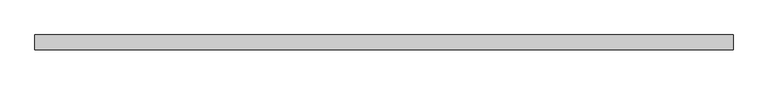
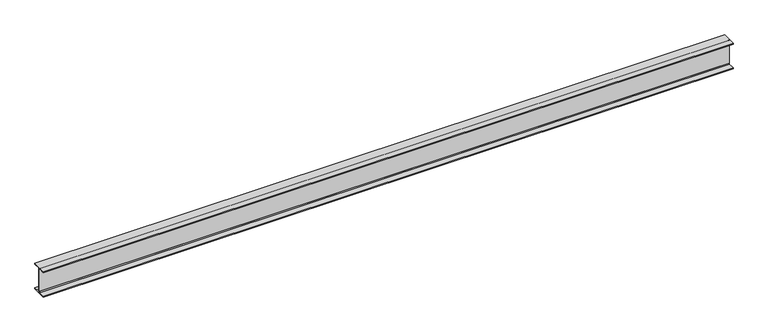
"""IFC4 building model written with IfcOpenShell, lengths in millimetres: beam geometry, Old_Steel Beam_H-KSD3502 : H_SB_ASB_H-300×300x10x15."""

from ifc_helpers import new_model, si_unit, point, frame, frame_2d, origin, place, context, project, spatial, polyline, circle_curve, trimmed, segment, composite_curve, outline, extrude, source, transform, mapped, element, save


def beam_0a0d776e(model_context):
    return source(origin(), model_context, "Body", "SweptSolid", [
        extrude(outline(composite_curve([segment(polyline([(82.5, -141.5), (82.5, -151.7), (-82.5, -151.7), (-82.5, -141.5), (-11.9, -141.5)]), True, "CONTINUOUS"), segment(trimmed(circle_curve(frame_2d((-11.9, -132.6)), 8.9), [point((-11.9, -141.5))], [point((-3.0, -132.6))], True, "CARTESIAN"), True, "CONTINUOUS"), segment(polyline([(-3.0, -132.6), (-3.0, 132.6)]), True, "CONTINUOUS"), segment(trimmed(circle_curve(frame_2d((-11.9, 132.6)), 8.9), [point((-3.0, 132.6))], [point((-11.9, 141.5))], True, "CARTESIAN"), True, "CONTINUOUS"), segment(polyline([(-11.9, 141.5), (-82.5, 141.5), (-82.5, 151.7), (82.5, 151.7), (82.5, 141.5), (11.9, 141.5)]), True, "CONTINUOUS"), segment(trimmed(circle_curve(frame_2d((11.9, 132.6)), 8.9), [point((11.9, 141.5))], [point((3.0, 132.6))], True, "CARTESIAN"), True, "CONTINUOUS"), segment(polyline([(3.0, 132.6), (3.0, -132.6)]), True, "CONTINUOUS"), segment(trimmed(circle_curve(frame_2d((11.9, -132.6)), 8.9), [point((3.0, -132.6))], [point((11.9, -141.5))], True, "CARTESIAN"), True, "CONTINUOUS"), segment(polyline([(11.9, -141.5), (82.5, -141.5)]), True, "CONTINUOUS")], self_intersect=False)), frame((-4027.4502484, 0.0, 0.0), z_axis=(1.0, 0.0, 0.0), x_axis=(0.0, 1.0, 0.0)), (0.0, 0.0, 1.0), 7805.3816456),
    ])


if __name__ == "__main__":
    model = new_model("IFC4")
    model_context = context("Model", 3, world=origin())
    ifc_project = project(units=[si_unit("LENGTHUNIT", "METRE", prefix="MILLI")], contexts=[model_context])
    site = spatial("IfcSite", under=ifc_project)
    building = spatial("IfcBuilding", under=site)
    placement = place(None, origin())
    beam_shape = beam_0a0d776e(model_context)
    element("IfcBeam", 1, ObjectType="Old_Steel Beam_H-KSD3502 : H_SB_ASB_H-300×300x10x15", at=placement, inside=building, context=model_context, shape_type="MappedRepresentation", body=[
        mapped(beam_shape, transform((0.0, 0.0, 0.0), x_axis=(1.0, 0.0, 0.0), y_axis=(0.0, 1.0, 0.0), z_axis=(0.0, 0.0, 1.0))),
    ])
    save(model, "model.ifc")

# Revit data of these elements
# Type "Old_Steel Beam_H-KSD3502 : H_SB_ASB_H-300×300x10x15"
#   Width = 30.0 cm
#   Web Thickness = 1.0 cm
#   Web Fillet = 1.8 cm
#   Warping Constant = 1370670.0 cm⁶
#   Torsional Moment of Inertia = 77.00 cm⁴
#   Torsional Modulus = 1.0 cm³
#   Section Area = 119.8 cm²
#   Plastic Modulus weak axis = 684.0 cm³
#   Plastic Modulus strong axis = 1500.0 cm³
#   Perimeter = 1.75 m²/m
#   Nominal Weight = 94.00 kgf/m
#   Moment of Inertia weak axis = 6750.00 cm⁴
#   Moment of Inertia strong axis = 20400.00 cm⁴
#   Height = 30.0 cm
#   Flange Thickness = 1.5 cm
#   Elastic Modulus weak axis = 450.0 cm³
#   Elastic Modulus strong axis = 1360.0 cm³
#   Centroid Vertical = 15.0 cm
#   Centroid Horizontal = 15.0 cm
#   Length [instance default] = 1.5240 m
#   Structural Material [instance default] = Steel, 45-345
#   Assembly Code = ""
# Element 1 (IfcBeam, "Old_Steel Beam_H-KSD3502 : H_SB_ASB_H-300×300x10x15")
#   Structural Material = none
# Materials
#   "Steel, 45-345": class "Metal", colour RGB 189 187 185, transparency 0, Description = "Steel 345 MPa", Cost = 0
